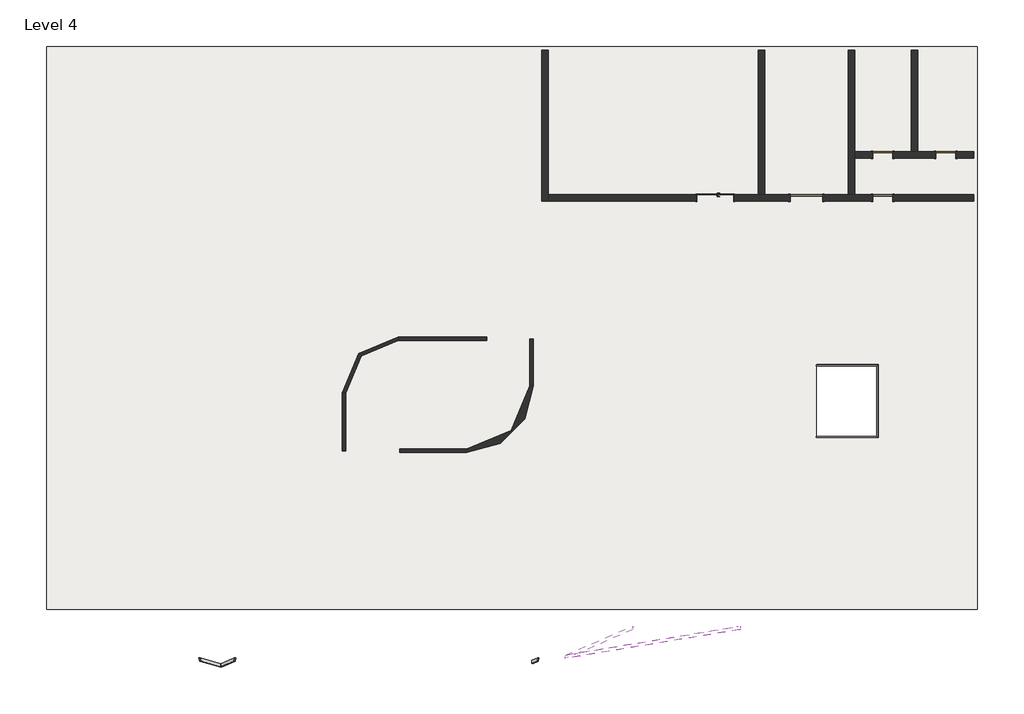
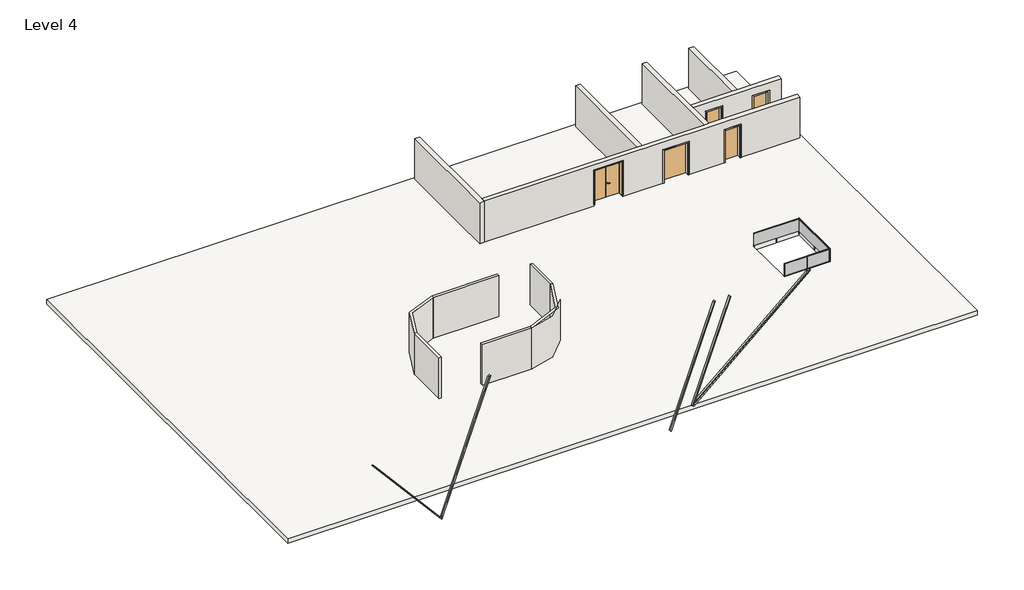
# One storey: 12 walls, 6 members, 5 doors, 1 railing, 1 slab.
"""IFC4 building model written with IfcOpenShell, lengths in millimetres."""

import ifcopenshell
import ifcopenshell.guid

model = None  # the IFC model being written
_history = None  # IfcOwnerHistory: only IFC2X3 demands one
_inside = {}  # id of a spatial element -> (the spatial element, [elements in it])
_under = {}  # id of a project, library or spatial element -> (it, [spatial elements below it])
_declared = {}  # id of a project -> (the project, [libraries it declares])
_typed = {}  # id of a type object -> (the type object, [elements of that type])
_made_of = {}  # id of a material, layer set ... -> (it, [elements and type objects made of it])


def new_model(schema):
    """Start an empty IFC model of exactly this schema.

    Asked for "IFC4X3", IfcOpenShell would pick the latest addendum, in which some entities
    have other attributes; the version numbers below select the first issue.
    IFC2X3 requires an IfcOwnerHistory on every rooted entity: one is made here for all.
    """
    global model, _history
    if schema == "IFC4X3":
        model = ifcopenshell.file(schema_version=(4, 3, 0, 0))
    else:
        model = ifcopenshell.file(schema=schema)
    _inside.clear()
    _under.clear()
    _declared.clear()
    _typed.clear()
    _made_of.clear()
    _history = None
    if model.schema == "IFC2X3":
        org = make("IfcOrganization", Name="unknown")
        user = make(
            "IfcPersonAndOrganization",
            ThePerson=make("IfcPerson", FamilyName="unknown"),
            TheOrganization=org,
        )
        app = make(
            "IfcApplication",
            ApplicationDeveloper=org,
            Version="unknown",
            ApplicationFullName="unknown",
            ApplicationIdentifier="unknown",
        )
        _history = make(
            "IfcOwnerHistory",
            OwningUser=user,
            OwningApplication=app,
            ChangeAction="ADDED",
            CreationDate=0,
        )
    return model


def make(cls, **values):
    """One entity of the class cls with the attributes given. An attribute that is None is left unset."""
    return model.create_entity(
        cls, **{name: value for name, value in values.items() if value is not None}
    )


def rooted(cls, **values):
    """An entity with a GlobalId (a new one), such as an element, a storey or a relation."""
    return make(cls, GlobalId=ifcopenshell.guid.new(), OwnerHistory=_history, **values)


def si_unit(unit_type, name, prefix=None):
    """IfcSIUnit, for example si_unit("LENGTHUNIT", "METRE", prefix="MILLI")."""
    return make("IfcSIUnit", UnitType=unit_type, Prefix=prefix, Name=name)


def assignment(units):
    """IfcUnitAssignment: the units of a project."""
    return None if units is None else make("IfcUnitAssignment", Units=units)


def point(xyz):
    """IfcCartesianPoint."""
    return None if xyz is None else make("IfcCartesianPoint", Coordinates=xyz)


def direction(xyz):
    """IfcDirection."""
    return None if xyz is None else make("IfcDirection", DirectionRatios=xyz)


def frame(location, z_axis=None, x_axis=None):
    """IfcAxis2Placement3D, a coordinate frame: its origin and axes. An axis left out is left unset."""
    return make(
        "IfcAxis2Placement3D",
        Location=point(location),
        Axis=direction(z_axis),
        RefDirection=direction(x_axis),
    )


def frame_2d(location, x_axis=None):
    """IfcAxis2Placement2D, a coordinate frame in the plane: its origin and x axis."""
    return make(
        "IfcAxis2Placement2D", Location=point(location), RefDirection=direction(x_axis)
    )


def origin():
    """The frame at (0, 0, 0) with its axes left unset."""
    return frame((0.0, 0.0, 0.0))


def origin_with_axes():
    """The frame at (0, 0, 0) with the z axis (0, 0, 1) and the x axis (1, 0, 0) written out."""
    return frame((0.0, 0.0, 0.0), z_axis=(0.0, 0.0, 1.0), x_axis=(1.0, 0.0, 0.0))


def place(relative_to, where):
    """IfcLocalPlacement: puts the frame where relative to a parent placement (None: the world)."""
    return make(
        "IfcLocalPlacement", PlacementRelTo=relative_to, RelativePlacement=where
    )


def context(
    kind, dimensions, precision=None, world=None, true_north=None, identifier=None
):
    """IfcGeometricRepresentationContext, for example the 3D "Model" context."""
    return make(
        "IfcGeometricRepresentationContext",
        ContextIdentifier=identifier,
        ContextType=kind,
        CoordinateSpaceDimension=dimensions,
        Precision=precision,
        WorldCoordinateSystem=world,
        TrueNorth=true_north,
    )


def project(units=None, contexts=None):
    """IfcProject with its units and contexts."""
    return rooted(
        "IfcProject",
        Name="project",
        RepresentationContexts=contexts,
        UnitsInContext=assignment(units),
    )


def spatial(cls, under=None, at=None, **own):
    """A site, building, storey or space (cls), placed at a placement, below another one or the project."""
    s = rooted(cls, ObjectPlacement=at, **own)
    if under is not None:
        _under.setdefault(under.id(), (under, []))[1].append(s)
    return s


def polyline(points):
    """IfcPolyline through the points."""
    return make("IfcPolyline", Points=[point(p) for p in points])


def circle_curve(where, radius):
    """IfcCircle in the frame where."""
    return make("IfcCircle", Position=where, Radius=radius)


def ellipse_curve(where, semi_axis1, semi_axis2):
    """IfcEllipse in the frame where."""
    return make(
        "IfcEllipse", Position=where, SemiAxis1=semi_axis1, SemiAxis2=semi_axis2
    )


def trimmed(basis, trim1, trim2, sense, master):
    """IfcTrimmedCurve: the piece of a basis curve between two trims."""
    return make(
        "IfcTrimmedCurve",
        BasisCurve=basis,
        Trim1=trim1,
        Trim2=trim2,
        SenseAgreement=sense,
        MasterRepresentation=master,
    )


def segment(curve, same_sense, transition):
    """IfcCompositeCurveSegment."""
    return make(
        "IfcCompositeCurveSegment",
        Transition=transition,
        SameSense=same_sense,
        ParentCurve=curve,
    )


def composite_curve(segments, self_intersect=None):
    """IfcCompositeCurve: segments joined end to end."""
    return make("IfcCompositeCurve", Segments=segments, SelfIntersect=self_intersect)


def outline(outer, holes=None, kind="AREA"):
    """IfcArbitraryClosedProfileDef: a profile drawn as a closed curve; with holes, ...WithVoids."""
    if holes is None:
        return make("IfcArbitraryClosedProfileDef", ProfileType=kind, OuterCurve=outer)
    return make(
        "IfcArbitraryProfileDefWithVoids",
        ProfileType=kind,
        OuterCurve=outer,
        InnerCurves=holes,
    )


def extrude(swept, where, along, depth):
    """IfcExtrudedAreaSolid: the profile swept, set in the frame where, extruded along a direction by depth."""
    return make(
        "IfcExtrudedAreaSolid",
        SweptArea=swept,
        Position=where,
        ExtrudedDirection=direction(along),
        Depth=depth,
    )


def faces_of(points, faces, orient=None, outer=None):
    """IfcFace entities. A face is a list of loops; a loop is a list of indices into points, from 0.

    orient and outer hold one flag for each loop. By default every Orientation is true, the
    first loop of a face is its IfcFaceOuterBound and the others are IfcFaceBound.
    """
    made = []
    for i, loops in enumerate(faces):
        bounds = []
        for j, loop in enumerate(loops):
            is_outer = j == 0 if outer is None else outer[i][j]
            bounds.append(
                make(
                    "IfcFaceOuterBound" if is_outer else "IfcFaceBound",
                    Bound=make("IfcPolyLoop", Polygon=[points[k] for k in loop]),
                    Orientation=True if orient is None else orient[i][j],
                )
            )
        made.append(make("IfcFace", Bounds=bounds))
    return made


def faceted_brep(points, faces, orient=None, outer=None, voids=None):
    """IfcFacetedBrep: a solid bounded by flat faces; with voids (closed shells), ...WithVoids."""
    shared = [point(p) for p in points]
    hull = make("IfcClosedShell", CfsFaces=faces_of(shared, faces, orient, outer))
    if voids is None:
        return make("IfcFacetedBrep", Outer=hull)
    return make(
        "IfcFacetedBrepWithVoids",
        Outer=hull,
        Voids=[
            make(cls, CfsFaces=faces_of(shared, fs, o, b)) for cls, fs, o, b in voids
        ],
    )


def shape(context_of_items, identifier, shape_type, items):
    """IfcShapeRepresentation: the items that make up one representation, for example the "Body"."""
    return make(
        "IfcShapeRepresentation",
        ContextOfItems=context_of_items,
        RepresentationIdentifier=identifier,
        RepresentationType=shape_type,
        Items=items,
    )


def source(mapping_origin, context_of_items, identifier, shape_type, items):
    """IfcRepresentationMap: a shape defined once, which mapped items show again and again."""
    return make(
        "IfcRepresentationMap",
        MappingOrigin=mapping_origin,
        MappedRepresentation=shape(context_of_items, identifier, shape_type, items),
    )


def transform(
    local_origin,
    x_axis=None,
    y_axis=None,
    z_axis=None,
    scale=None,
    scale2=None,
    scale3=None,
    uniform=True,
):
    """IfcCartesianTransformationOperator3D, or its non-uniform kind. x_axis, y_axis, z_axis: its Axis1, 2, 3."""
    if uniform:
        return make(
            "IfcCartesianTransformationOperator3D",
            Axis1=direction(x_axis),
            Axis2=direction(y_axis),
            LocalOrigin=point(local_origin),
            Scale=scale,
            Axis3=direction(z_axis),
        )
    return make(
        "IfcCartesianTransformationOperator3DnonUniform",
        Axis1=direction(x_axis),
        Axis2=direction(y_axis),
        LocalOrigin=point(local_origin),
        Scale=scale,
        Axis3=direction(z_axis),
        Scale2=scale2,
        Scale3=scale3,
    )


def mapped(mapping_source, mapping_target):
    """IfcMappedItem: shows the shape of a source again, moved by a transform."""
    return make(
        "IfcMappedItem", MappingSource=mapping_source, MappingTarget=mapping_target
    )


def made_of(thing, what):
    """Note that an element or type object is made of a material, layer set ...; save() writes the relation."""
    if what is not None:
        _made_of.setdefault(what.id(), (what, []))[1].append(thing)
    return thing


def element(
    cls,
    number,
    at=None,
    inside=None,
    cuts=None,
    type_object=None,
    material=None,
    context=None,
    identifier="Body",
    shape_type=None,
    held_by="IfcProductDefinitionShape",
    body=None,
    shapes=None,
    **own,
):
    """One element of the class cls, such as IfcWall. Its Tag is "e" and its number.

    at: its placement. inside: the storey or other place that contains it. cuts: it is an
    opening in that element (IfcRelVoidsElement). A single representation is given by context,
    identifier, shape_type and body (its items); several are given by shapes. held_by: the class
    of the entity that holds the representations. save() writes the other relations.
    """
    e = rooted(cls, Tag="e%d" % number, ObjectPlacement=at, **own)
    if body is not None:
        shapes = [shape(context, identifier, shape_type, body)]
    if shapes is not None:
        e.Representation = make(held_by, Representations=shapes)
    if inside is not None:
        _inside.setdefault(inside.id(), (inside, []))[1].append(e)
    if cuts is not None:
        rooted(
            "IfcRelVoidsElement", RelatingBuildingElement=cuts, RelatedOpeningElement=e
        )
    if type_object is not None:
        _typed.setdefault(type_object.id(), (type_object, []))[1].append(e)
    return made_of(e, material)


def aggregate(whole, parts):
    """IfcRelAggregates: a whole, such as a stair, and the parts it consists of."""
    return rooted("IfcRelAggregates", RelatingObject=whole, RelatedObjects=parts)


def save(model, path):
    """Write the relations noted so far, then the file.

    IfcRelAggregates (storeys below a building ...), IfcRelContainedInSpatialStructure (elements
    in a storey), IfcRelDefinesByType, IfcRelAssociatesMaterial and IfcRelDeclares: one each for
    every whole, place, type object, material and project.
    """
    for whole, parts in _under.values():
        aggregate(whole, parts)
    for where, things in _inside.values():
        rooted(
            "IfcRelContainedInSpatialStructure",
            RelatedElements=things,
            RelatingStructure=where,
        )
    for kind, things in _typed.values():
        rooted("IfcRelDefinesByType", RelatedObjects=things, RelatingType=kind)
    for what, things in _made_of.values():
        rooted("IfcRelAssociatesMaterial", RelatedObjects=things, RelatingMaterial=what)
    for by, libraries in _declared.values():
        rooted("IfcRelDeclares", RelatingContext=by, RelatedDefinitions=libraries)
    model.write(path)


def plane_surface(at):
    """IfcPlane: the flat surface through the origin of the frame at, square to its z axis."""
    return make("IfcPlane", Position=at)


def cylinder_surface(at, radius):
    """IfcCylindricalSurface: all points at the distance radius from the z axis of the frame at."""
    return make("IfcCylindricalSurface", Position=at, Radius=radius)


def advanced_brep(points, edges, surfaces, faces):
    """IfcAdvancedBrep: a solid bounded by faces that lie on surfaces and meet in shared edges.

    An edge is (start, end): straight between two places in points (the first is 0);
    or (start, end, curve); or (start, end, curve, False) where it runs against its curve.
    A face is (place in surfaces, loops), or (place, loops, False) where it looks against
    its surface's normal. A loop lists edges by number (the first is 1), with a minus sign
    where the edge is run from its end to its start. The first loop is the outer one.
    """
    corners = [point(p) for p in points]
    vertices = [make("IfcVertexPoint", VertexGeometry=c) for c in corners]
    made = []
    for start, end, *more in edges:
        made.append(
            make(
                "IfcEdgeCurve",
                EdgeStart=vertices[start],
                EdgeEnd=vertices[end],
                EdgeGeometry=more[0] if more else make("IfcPolyline", Points=[corners[start], corners[end]]),
                SameSense=more[1] if len(more) > 1 else True,
            )
        )
    hull = []
    for where, loops, *sense in faces:
        bounds = []
        for j, loop in enumerate(loops):
            ring = [make("IfcOrientedEdge", EdgeElement=made[abs(k) - 1], Orientation=k > 0) for k in loop]
            bounds.append(
                make(
                    "IfcFaceOuterBound" if j == 0 else "IfcFaceBound",
                    Bound=make("IfcEdgeLoop", EdgeList=ring),
                    Orientation=True,
                )
            )
        hull.append(make("IfcAdvancedFace", Bounds=bounds, FaceSurface=surfaces[where], SameSense=sense[0] if sense else True))
    return make("IfcAdvancedBrep", Outer=make("IfcClosedShell", CfsFaces=hull))


def door_double_flush_variable_door_double_flush_variable_ac6c3b87(model_context):
    return source(origin(), model_context, "Body", "SolidModel", [
        advanced_brep(
        [(90.0, 139.4346141, 1000.0), (110.0, 139.4346141, 1000.0), (90.0, 69.4346141, 1000.0), (110.0, 89.4346141, 1000.0), (220.0, 69.4346141, 1000.0), (220.0, 89.4346141, 1000.0)],
        [
            (0, 1, circle_curve(frame((100.0, 139.4346141, 1000.0), z_axis=(0.0, 1.0, 0.0), x_axis=(1.0, 0.0, 0.0)), 10.0)),
            (1, 0, circle_curve(frame((100.0, 139.4346141, 1000.0), z_axis=(0.0, 1.0, 0.0), x_axis=(1.0, 0.0, 0.0)), 10.0)),
            (0, 2),
            (2, 3, ellipse_curve(frame((100.0, 79.4346141, 1000.0), z_axis=(-0.7071067811865385, 0.7071067811865565, 0.0), x_axis=(0.7071067811865563, 0.7071067811865386, 0.0)), 14.1421356, 10.0)),
            (3, 1),
            (3, 2, ellipse_curve(frame((100.0, 79.4346141, 1000.0), z_axis=(-0.7071067811865385, 0.7071067811865565, 0.0), x_axis=(0.7071067811865563, 0.7071067811865386, 0.0)), 14.1421356, 10.0)),
            (4, 5, circle_curve(frame((220.0, 79.4346141, 1000.0), z_axis=(1.0, 0.0, 0.0), x_axis=(0.0, 1.0, 0.0)), 10.0)),
            (5, 4, circle_curve(frame((220.0, 79.4346141, 1000.0), z_axis=(1.0, 0.0, 0.0), x_axis=(0.0, 1.0, 0.0)), 10.0)),
            (2, 4),
            (5, 3),
        ],
        [
            plane_surface(frame((100.0, 139.4346141, -287.7526403), z_axis=(0.0, 1.0, 0.0), x_axis=(0.0, 0.0, 1.0))),
            cylinder_surface(frame((100.0, 139.4346141, 1000.0), z_axis=(0.0, 1.0, 0.0), x_axis=(1.0, 0.0, 0.0)), 10.0),
            plane_surface(frame((220.0, 79.4346141, -287.7526403), z_axis=(1.0, 0.0, 0.0), x_axis=(0.0, 0.0, 1.0))),
            cylinder_surface(frame((100.0, 79.4346141, 1000.0), z_axis=(-1.0, 0.0, 0.0), x_axis=(0.0, 1.0, 0.0)), 10.0),
        ],
        [
            (0, [[1, 2]]),
            (1, [[-1, 3, 4, 5]]),
            (1, [[-2, -5, 6, -3]]),
            (2, [[7, 8]]),
            (3, [[-4, 9, -8, 10]]),
            (3, [[-6, -10, -7, -9]]),
        ],
    ),
        advanced_brep(
        [(110.0, 199.4346141, 1000.0), (90.0, 199.4346141, 1000.0), (110.0, 229.4346141, 1000.0), (90.0, 249.4346141, 1000.0), (220.0, 229.4346141, 1000.0), (220.0, 249.4346141, 1000.0)],
        [
            (0, 1, circle_curve(frame((100.0, 199.4346141, 1000.0), z_axis=(0.0, -1.0, 0.0), x_axis=(-1.0, 0.0, 0.0)), 10.0)),
            (1, 0, circle_curve(frame((100.0, 199.4346141, 1000.0), z_axis=(0.0, -1.0, 0.0), x_axis=(-1.0, 0.0, 0.0)), 10.0)),
            (0, 2),
            (2, 3, ellipse_curve(frame((100.0, 239.4346141, 1000.0), z_axis=(-0.7071067811865475, -0.7071067811865475, 0.0), x_axis=(0.7071067811865474, -0.7071067811865476, 0.0)), 14.1421356, 10.0)),
            (3, 1),
            (3, 2, ellipse_curve(frame((100.0, 239.4346141, 1000.0), z_axis=(-0.7071067811865475, -0.7071067811865475, 0.0), x_axis=(0.7071067811865474, -0.7071067811865476, 0.0)), 14.1421356, 10.0)),
            (4, 5, circle_curve(frame((220.0, 239.4346141, 1000.0), z_axis=(1.0, 0.0, 0.0), x_axis=(0.0, 1.0, 0.0)), 10.0)),
            (5, 4, circle_curve(frame((220.0, 239.4346141, 1000.0), z_axis=(1.0, 0.0, 0.0), x_axis=(0.0, 1.0, 0.0)), 10.0)),
            (2, 4),
            (5, 3),
        ],
        [
            plane_surface(frame((100.0, 199.4346141, -287.7526403), z_axis=(0.0, -1.0, 0.0), x_axis=(0.0, 0.0, 1.0))),
            cylinder_surface(frame((100.0, 199.4346141, 1000.0), z_axis=(0.0, -1.0, 0.0), x_axis=(-1.0, 0.0, 0.0)), 10.0),
            plane_surface(frame((220.0, 239.4346141, -287.7526403), z_axis=(1.0, 0.0, 0.0), x_axis=(0.0, 0.0, 1.0))),
            cylinder_surface(frame((100.0, 239.4346141, 1000.0), z_axis=(-1.0, 0.0, 0.0), x_axis=(0.0, 1.0, 0.0)), 10.0),
        ],
        [
            (0, [[1, 2]]),
            (1, [[-1, 3, 4, 5]]),
            (1, [[-2, -5, 6, -3]]),
            (2, [[7, 8]]),
            (3, [[-4, 9, -8, 10]]),
            (3, [[-6, -10, -7, -9]]),
        ],
    ),
        extrude(outline(composite_curve([segment(trimmed(circle_curve(frame_2d((1000.0, 100.0)), 20.0), [point((1000.0, 80.0))], [point((1000.0, 120.0))], False, "CARTESIAN"), True, "CONTINUOUS"), segment(trimmed(circle_curve(frame_2d((1000.0, 100.0)), 20.0), [point((1000.0, 120.0))], [point((1000.0, 80.0))], False, "CARTESIAN"), True, "CONTINUOUS")], self_intersect=False)), frame((0.0, 129.4346141, 0.0), z_axis=(0.0, 1.0, 0.0), x_axis=(0.0, 0.0, 1.0)), (0.0, 0.0, 1.0), 10.0),
        extrude(outline(composite_curve([segment(trimmed(circle_curve(frame_2d((1000.0, 100.0)), 20.0), [point((1000.0, 80.0))], [point((1000.0, 120.0))], False, "CARTESIAN"), True, "CONTINUOUS"), segment(trimmed(circle_curve(frame_2d((1000.0, 100.0)), 20.0), [point((1000.0, 120.0))], [point((1000.0, 80.0))], False, "CARTESIAN"), True, "CONTINUOUS")], self_intersect=False)), frame((0.0, 189.4346141, 0.0), z_axis=(0.0, 1.0, 0.0), x_axis=(0.0, 0.0, 1.0)), (0.0, 0.0, 1.0), 10.0),
        extrude(outline(polyline([(0.0, 164.4346141), (-871.25, 164.4346141), (-871.25, 189.4346141), (0.0, 189.4346141), (0.0, 164.4346141)])), frame((0.0, 0.0, 100.0), z_axis=(0.0, 0.0, 1.0), x_axis=(1.0, 0.0, 0.0)), (0.0, 0.0, 1.0), 2250.0),
        extrude(outline(polyline([(871.25, 164.4346141), (0.0, 164.4346141), (0.0, 189.4346141), (871.25, 189.4346141), (871.25, 164.4346141)])), frame((0.0, 0.0, 100.0), z_axis=(0.0, 0.0, 1.0), x_axis=(1.0, 0.0, 0.0)), (0.0, 0.0, 1.0), 2250.0),
        faceted_brep([(905.75, -150.5653859, 100.0), (856.25, -150.5653859, 100.0), (856.25, 164.4346141, 100.0), (871.25, 164.4346141, 100.0), (871.25, 189.4346141, 100.0), (905.75, 189.4346141, 100.0), (905.75, 164.4346141, 100.0), (900.75, 164.4346141, 100.0), (900.75, 184.4346141, 100.0), (876.25, 184.4346141, 100.0), (876.25, 159.4346141, 100.0), (861.25, 159.4346141, 100.0), (861.25, -145.5653859, 100.0), (900.75, -145.5653859, 100.0), (900.75, -135.5653859, 100.0), (905.75, -135.5653859, 100.0), (905.75, -150.5653859, 2384.5), (-905.75, -150.5653859, 2384.5), (-905.75, -150.5653859, 100.0), (-856.25, -150.5653859, 100.0), (-856.25, -150.5653859, 2335.0), (856.25, -150.5653859, 2335.0), (856.25, 164.4346141, 2335.0), (-856.25, 164.4346141, 2335.0), (-856.25, 164.4346141, 100.0), (-871.25, 164.4346141, 100.0), (-871.25, 164.4346141, 2350.0), (871.25, 164.4346141, 2350.0), (871.25, 189.4346141, 2350.0), (-871.25, 189.4346141, 2350.0), (-871.25, 189.4346141, 100.0), (-905.75, 189.4346141, 100.0), (-905.75, 189.4346141, 2384.5), (905.75, 189.4346141, 2384.5), (905.75, 164.4346141, 2384.5), (-905.75, 164.4346141, 2384.5), (-905.75, 164.4346141, 100.0), (-900.75, 164.4346141, 100.0), (-900.75, 164.4346141, 2379.5), (900.75, 164.4346141, 2379.5), (900.75, 184.4346141, 2379.5), (-900.75, 184.4346141, 2379.5), (-900.75, 184.4346141, 100.0), (-876.25, 184.4346141, 100.0), (-876.25, 184.4346141, 2355.0), (876.25, 184.4346141, 2355.0), (876.25, 159.4346141, 2355.0), (-876.25, 159.4346141, 2355.0), (-876.25, 159.4346141, 100.0), (-861.25, 159.4346141, 100.0), (-861.25, 159.4346141, 2340.0), (861.25, 159.4346141, 2340.0), (861.25, -145.5653859, 2340.0), (-861.25, -145.5653859, 2340.0), (-861.25, -145.5653859, 100.0), (-900.75, -145.5653859, 100.0), (-900.75, -145.5653859, 2379.5), (900.75, -145.5653859, 2379.5), (900.75, -135.5653859, 2379.5), (-900.75, -135.5653859, 2379.5), (-900.75, -135.5653859, 100.0), (-905.75, -135.5653859, 100.0), (-905.75, -135.5653859, 2384.5), (905.75, -135.5653859, 2384.5)], [[[0, 1, 2, 3, 4, 5, 6, 7, 8, 9, 10, 11, 12, 13, 14, 15]], [[1, 0, 16, 17, 18, 19, 20, 21]], [[2, 1, 21, 22]], [[3, 2, 22, 23, 24, 25, 26, 27]], [[4, 3, 27, 28]], [[5, 4, 28, 29, 30, 31, 32, 33]], [[6, 5, 33, 34]], [[7, 6, 34, 35, 36, 37, 38, 39]], [[8, 7, 39, 40]], [[9, 8, 40, 41, 42, 43, 44, 45]], [[10, 9, 45, 46]], [[11, 10, 46, 47, 48, 49, 50, 51]], [[12, 11, 51, 52]], [[13, 12, 52, 53, 54, 55, 56, 57]], [[14, 13, 57, 58]], [[15, 14, 58, 59, 60, 61, 62, 63]], [[0, 15, 63, 16]], [[17, 62, 61, 18]], [[18, 61, 60, 55, 54, 49, 48, 43, 42, 37, 36, 31, 30, 25, 24, 19]], [[23, 20, 19, 24]], [[29, 26, 25, 30]], [[35, 32, 31, 36]], [[41, 38, 37, 42]], [[47, 44, 43, 48]], [[53, 50, 49, 54]], [[59, 56, 55, 60]], [[22, 21, 20, 23]], [[28, 27, 26, 29]], [[34, 33, 32, 35]], [[40, 39, 38, 41]], [[46, 45, 44, 47]], [[52, 51, 50, 53]], [[58, 57, 56, 59]], [[16, 63, 62, 17]]]),
    ])


def m_single_flush_0915_x_2134mm_1c84716f(model_context):
    return source(origin(), model_context, "Body", "SweptSolid", [
        extrude(outline(polyline([(2210.0, -533.5), (0.0, -533.5), (0.0, -457.5), (2134.0, -457.5), (2134.0, 457.5), (0.0, 457.5), (0.0, 533.5), (2210.0, 533.5), (2210.0, -533.5)])), frame((0.0, -175.0, 0.0), z_axis=(0.0, 1.0, 0.0), x_axis=(0.0, 0.0, 1.0)), (0.0, 0.0, 1.0), 25.0),
        extrude(outline(polyline([(2210.0, 533.5), (2210.0, -533.5), (0.0, -533.5), (0.0, -457.5), (2134.0, -457.5), (2134.0, 457.5), (0.0, 457.5), (0.0, 533.5), (2210.0, 533.5)])), frame((0.0, 150.0, 0.0), z_axis=(0.0, 1.0, 0.0), x_axis=(0.0, 0.0, 1.0)), (0.0, 0.0, 1.0), 25.0),
        extrude(outline(polyline([(457.5, -99.0), (457.5, -150.0), (-457.5, -150.0), (-457.5, -99.0), (457.5, -99.0)])), origin_with_axes(), (0.0, 0.0, 1.0), 2134.0),
    ])


def m_single_flush_1500_x_2134mm_2_edebd810(model_context):
    return source(origin(), model_context, "Body", "SweptSolid", [
        extrude(outline(polyline([(2210.0, -826.0), (0.0, -826.0), (0.0, -750.0), (2134.0, -750.0), (2134.0, 750.0), (0.0, 750.0), (0.0, 826.0), (2210.0, 826.0), (2210.0, -826.0)])), frame((0.0, -175.0, 0.0), z_axis=(0.0, 1.0, 0.0), x_axis=(0.0, 0.0, 1.0)), (0.0, 0.0, 1.0), 25.0),
        extrude(outline(polyline([(2210.0, 826.0), (2210.0, -826.0), (0.0, -826.0), (0.0, -750.0), (2134.0, -750.0), (2134.0, 750.0), (0.0, 750.0), (0.0, 826.0), (2210.0, 826.0)])), frame((0.0, 150.0, 0.0), z_axis=(0.0, 1.0, 0.0), x_axis=(0.0, 0.0, 1.0)), (0.0, 0.0, 1.0), 25.0),
        extrude(outline(polyline([(750.0, -99.0), (750.0, -150.0), (-750.0, -150.0), (-750.0, -99.0), (750.0, -99.0)])), origin_with_axes(), (0.0, 0.0, 1.0), 2134.0),
    ])


def rectangular_mullion_50_x_150mm_6888afb9(model_context):
    return source(origin(), model_context, "Body", "SweptSolid", [
        extrude(outline(polyline([(0.0, 0.0), (-85.321119, -50.0), (-8217.0308307, -50.0), (-8288.6527046, 0.0), (0.0, 0.0)])), frame((0.0, -75.0, 0.0), z_axis=(0.0, 1.0, 0.0), x_axis=(0.0, 0.0, 1.0)), (0.0, 0.0, 1.0), 150.0),
    ])


def rectangular_mullion_50_x_150mm_7805e086(model_context):
    return source(origin(), model_context, "Body", "SweptSolid", [
        extrude(outline(polyline([(0.0, 0.0), (-85.321119, -50.0), (-7488.5336568, -50.0), (-7500.253691, 0.0), (0.0, 0.0)])), frame((0.0, -75.0, 0.0), z_axis=(0.0, 1.0, 0.0), x_axis=(0.0, 0.0, 1.0)), (0.0, 0.0, 1.0), 150.0),
    ])


def rectangular_mullion_50_x_150mm_3e1f935b(model_context):
    return source(origin(), model_context, "Body", "SweptSolid", [
        extrude(outline(polyline([(0.0, 0.0), (-213.3099575, -50.0), (-6299.3378645, -50.0), (-6328.6389336, 0.0), (0.0, 0.0)])), frame((0.0, -75.0, 0.0), z_axis=(0.0, 1.0, 0.0), x_axis=(0.0, 0.0, 1.0)), (0.0, 0.0, 1.0), 150.0),
    ])


def rectangular_mullion_50_x_150mm_2c60866a(model_context):
    return source(origin(), model_context, "Body", "SweptSolid", [
        extrude(outline(polyline([(0.0, 0.0), (-71.6218739, -50.0), (-5613.3621531, -50.0), (-5648.2676905, 0.0), (0.0, 0.0)])), frame((0.0, -75.0, 0.0), z_axis=(0.0, 1.0, 0.0), x_axis=(0.0, 0.0, 1.0)), (0.0, 0.0, 1.0), 150.0),
    ])


def rectangular_mullion_50_x_150mm_3d64617b(model_context):
    return source(origin(), model_context, "Body", "SweptSolid", [
        extrude(outline(polyline([(0.0, 0.0), (-11.7094446, -50.0), (-9724.6362561, -50.0), (-9783.1614006, 0.0), (0.0, 0.0)])), frame((0.0, -75.0, 0.0), z_axis=(0.0, 1.0, 0.0), x_axis=(0.0, 0.0, 1.0)), (0.0, 0.0, 1.0), 150.0),
    ])


def rectangular_mullion_50_x_150mm_375b3459(model_context):
    return source(origin(), model_context, "Body", "SweptSolid", [
        extrude(outline(polyline([(0.0, 0.0), (-161.7316361, -50.0), (-9569.8514431, -50.0), (-9783.1614006, 0.0), (0.0, 0.0)])), frame((0.0, -75.0, 0.0), z_axis=(0.0, 1.0, 0.0), x_axis=(0.0, 0.0, 1.0)), (0.0, 0.0, 1.0), 150.0),
    ])


def glas_mpk_39525c5c(model_context):
    return source(origin(), model_context, "Body", "SolidModel", [
        faceted_brep([(28810.8437289, 1285.374085, 9843.2628643), (28810.8437289, 1235.374085, 9843.2628643), (28810.8437289, 1235.374085, 9856.7371357), (28810.8437289, 1285.374085, 9856.7371357), (31650.8437289, 1285.374085, 9843.2628643), (31600.8437289, 1235.374085, 9843.2628643), (31600.8437289, 1235.374085, 9856.7371357), (31650.8437289, 1285.374085, 9856.7371357), (31650.8437289, -2055.3552612, 9843.2628643), (31600.8437289, -2005.3552612, 9843.2628643), (31600.8437289, -2005.3552612, 9856.7371357), (31650.8437289, -2055.3552612, 9856.7371357), (28810.8437289, -2055.3552612, 9843.2628643), (28810.8437289, -2055.3552612, 9856.7371357), (28810.8437289, -2005.3552612, 9856.7371357), (28810.8437289, -2005.3552612, 9843.2628643)], [[[0, 1, 2, 3]], [[1, 0, 4, 5]], [[2, 1, 5, 6]], [[3, 2, 6, 7]], [[0, 3, 7, 4]], [[5, 4, 8, 9]], [[6, 5, 9, 10]], [[7, 6, 10, 11]], [[4, 7, 11, 8]], [[12, 13, 14, 15]], [[9, 8, 12, 15]], [[10, 9, 15, 14]], [[11, 10, 14, 13]], [[8, 11, 13, 12]]]),
        faceted_brep([(28810.8437289, 1245.374085, 9842.8769824), (28810.8437289, 1259.566209, 9842.8769824), (28810.8437289, 1259.566209, 9042.8769824), (28810.8437289, 1245.374085, 9042.8769824), (31610.8437289, 1245.374085, 9842.8769824), (31625.0358529, 1259.566209, 9842.8769824), (31625.0358529, 1259.566209, 9042.8769824), (31610.8437289, 1245.374085, 9042.8769824), (31610.8437289, -2015.3552612, 9842.8769824), (31625.0358529, -2029.5473852, 9842.8769824), (31625.0358529, -2029.5473852, 9042.8769824), (31610.8437289, -2015.3552612, 9042.8769824), (28810.8437289, -2015.3552612, 9842.8769824), (28810.8437289, -2015.3552612, 9042.8769824), (28810.8437289, -2029.5473852, 9042.8769824), (28810.8437289, -2029.5473852, 9842.8769824)], [[[0, 1, 2, 3]], [[1, 0, 4, 5]], [[2, 1, 5, 6]], [[3, 2, 6, 7]], [[0, 3, 7, 4]], [[5, 4, 8, 9]], [[6, 5, 9, 10]], [[7, 6, 10, 11]], [[4, 7, 11, 8]], [[12, 13, 14, 15]], [[9, 8, 12, 15]], [[10, 9, 15, 14]], [[11, 10, 14, 13]], [[8, 11, 13, 12]]]),
        extrude(outline(polyline([(30242.0937289, -2030.3552612), (30242.0937289, -2055.3552612), (30217.0937289, -2055.3552612), (30217.0937289, -2030.3552612), (30242.0937289, -2030.3552612)])), frame((0.0, 0.0, 8800.0), z_axis=(0.0, 0.0, 1.0), x_axis=(1.0, 0.0, 0.0)), (0.0, 0.0, 1.0), 1043.2628643),
        extrude(outline(polyline([(31625.8437289, -372.4905881), (31650.8437289, -372.4905881), (31650.8437289, -397.4905881), (31625.8437289, -397.4905881), (31625.8437289, -372.4905881)])), frame((0.0, 0.0, 8800.0), z_axis=(0.0, 0.0, 1.0), x_axis=(1.0, 0.0, 0.0)), (0.0, 0.0, 1.0), 1043.2628643),
        extrude(outline(polyline([(30217.0937289, 1260.374085), (30217.0937289, 1285.374085), (30242.0937289, 1285.374085), (30242.0937289, 1260.374085), (30217.0937289, 1260.374085)])), frame((0.0, 0.0, 8800.0), z_axis=(0.0, 0.0, 1.0), x_axis=(1.0, 0.0, 0.0)), (0.0, 0.0, 1.0), 1043.2628643),
        extrude(outline(polyline([(31625.8437289, -2040.3552612), (31650.8437289, -2040.3552612), (31650.8437289, -2065.3552612), (31625.8437289, -2065.3552612), (31625.8437289, -2040.3552612)])), frame((0.0, 0.0, 8800.0), z_axis=(0.0, 0.0, 1.0), x_axis=(1.0, 0.0, 0.0)), (0.0, 0.0, 1.0), 1043.2628643),
        extrude(outline(polyline([(31635.8437289, 1260.374085), (31635.8437289, 1285.374085), (31660.8437289, 1285.374085), (31660.8437289, 1260.374085), (31635.8437289, 1260.374085)])), frame((0.0, 0.0, 8800.0), z_axis=(0.0, 0.0, 1.0), x_axis=(1.0, 0.0, 0.0)), (0.0, 0.0, 1.0), 1043.2628643),
        extrude(outline(polyline([(28823.3437289, -2030.3552612), (28823.3437289, -2055.3552612), (28798.3437289, -2055.3552612), (28798.3437289, -2030.3552612), (28823.3437289, -2030.3552612)])), frame((0.0, 0.0, 8800.0), z_axis=(0.0, 0.0, 1.0), x_axis=(1.0, 0.0, 0.0)), (0.0, 0.0, 1.0), 1043.2628643),
        extrude(outline(polyline([(28810.8437289, 1260.374085), (28810.8437289, 1285.374085), (28835.8437289, 1285.374085), (28835.8437289, 1260.374085), (28810.8437289, 1260.374085)])), frame((0.0, 0.0, 8800.0), z_axis=(0.0, 0.0, 1.0), x_axis=(1.0, 0.0, 0.0)), (0.0, 0.0, 1.0), 1043.2628643),
    ])


model = new_model("IFC4")

# Units and contexts
model_context = context("Model", 3, world=origin())
ifc_project = project(units=[si_unit("LENGTHUNIT", "METRE", prefix="MILLI")], contexts=[model_context])

# Site, building, storey
site = spatial("IfcSite", under=ifc_project)
building = spatial("IfcBuilding", under=site)
storey = spatial("IfcBuildingStorey", under=building, Name="Level 4", Elevation=9000.0)

# Doors
placement = place(None, origin())
door_double_flush_variable_door_double_flush_variable_shape = door_double_flush_variable_door_double_flush_variable_ac6c3b87(model_context)
element("IfcDoor", 1, ObjectType="Door Double Flush - Variable : Door Double Flush - Variable", at=placement, inside=storey, context=model_context, shape_type="MappedRepresentation", body=[
    mapped(door_double_flush_variable_door_double_flush_variable_shape, transform((24136.7471367, 8984.3231089, 9000.0), x_axis=(1.0, 0.0, 0.0), y_axis=(0.0, 1.0, 0.0), z_axis=(0.0, 0.0, 1.0))),
])
m_single_flush_0915_x_2134mm_shape = m_single_flush_0915_x_2134mm_1c84716f(model_context)
element("IfcDoor", 2, ObjectType="M_Single-Flush : 0915 x 2134mm", at=placement, inside=storey, context=model_context, shape_type="MappedRepresentation", body=[
    mapped(m_single_flush_0915_x_2134mm_shape, transform((34787.1221367, 10998.757723, 9000.0), x_axis=(-1.0, 0.0, 0.0), y_axis=(0.0, -1.0, 0.0), z_axis=(0.0, 0.0, 1.0))),
])
element("IfcDoor", 3, ObjectType="M_Single-Flush : 0915 x 2134mm", at=placement, inside=storey, context=model_context, shape_type="MappedRepresentation", body=[
    mapped(m_single_flush_0915_x_2134mm_shape, transform((31874.3721367, 10998.757723, 9000.0), x_axis=(-1.0, 0.0, 0.0), y_axis=(0.0, -1.0, 0.0), z_axis=(0.0, 0.0, 1.0))),
])
element("IfcDoor", 4, ObjectType="M_Single-Flush : 0915 x 2134mm", at=placement, inside=storey, context=model_context, shape_type="MappedRepresentation", body=[
    mapped(m_single_flush_0915_x_2134mm_shape, transform((31874.3721367, 8998.757723, 9000.0), x_axis=(-1.0, 0.0, 0.0), y_axis=(0.0, -1.0, 0.0), z_axis=(0.0, 0.0, 1.0))),
])
m_single_flush_1500_x_2134mm_2_shape = m_single_flush_1500_x_2134mm_2_edebd810(model_context)
element("IfcDoor", 5, ObjectType="M_Single-Flush : 1500 x 2134mm 2", at=placement, inside=storey, context=model_context, shape_type="MappedRepresentation", body=[
    mapped(m_single_flush_1500_x_2134mm_2_shape, transform((28342.9971367, 8998.757723, 9000.0), x_axis=(-1.0, 0.0, 0.0), y_axis=(0.0, -1.0, 0.0), z_axis=(0.0, 0.0, 1.0))),
])

# Members
rectangular_mullion_50_x_150mm_shape = rectangular_mullion_50_x_150mm_6888afb9(model_context)
element("IfcMember", 6, ObjectType="Rectangular Mullion : 50 x 150mm", at=placement, inside=storey, context=model_context, shape_type="MappedRepresentation", body=[
    mapped(rectangular_mullion_50_x_150mm_shape, transform((5377.8841529, -10856.2576342, 16077.9460567), x_axis=(0.8724314351462178, -0.11823606660145622, -0.4742189615813849), y_axis=(0.0, 0.9702957262759964, -0.24192189559966842), z_axis=(0.48873652510193155, 0.21106026657131102, 0.8465164929912093))),
])
rectangular_mullion_50_x_150mm_2_shape = rectangular_mullion_50_x_150mm_7805e086(model_context)
element("IfcMember", 7, ObjectType="Rectangular Mullion : 50 x 150mm", at=placement, inside=storey, context=model_context, shape_type="MappedRepresentation", body=[
    mapped(rectangular_mullion_50_x_150mm_2_shape, transform((19377.8841529, -10856.2576342, 16077.9460567), x_axis=(0.8724314351462182, -0.118236066601456, -0.474218961581384), y_axis=(0.0, 0.9702957262759963, -0.24192189559966853), z_axis=(0.48873652510193055, 0.21106026657131124, 0.8465164929912097))),
])
rectangular_mullion_50_x_150mm_3_shape = rectangular_mullion_50_x_150mm_3e1f935b(model_context)
element("IfcMember", 8, ObjectType="Rectangular Mullion : 50 x 150mm", at=placement, inside=storey, context=model_context, shape_type="MappedRepresentation", body=[
    mapped(rectangular_mullion_50_x_150mm_3_shape, transform((17207.380392, -12191.9818546, 10720.6488212), x_axis=(-0.8724314351462175, 0.11823606660145633, 0.4742189615813853), y_axis=(0.0, 0.9702957262759964, -0.2419218955996684), z_axis=(-0.488736525101932, -0.21106026657131094, -0.8465164929912091))),
])
rectangular_mullion_50_x_150mm_4_shape = rectangular_mullion_50_x_150mm_2c60866a(model_context)
element("IfcMember", 9, ObjectType="Rectangular Mullion : 50 x 150mm", at=placement, inside=storey, context=model_context, shape_type="MappedRepresentation", body=[
    mapped(rectangular_mullion_50_x_150mm_4_shape, transform((1326.9168323, -12605.6628836, 9061.4648376), x_axis=(-0.7594865733990562, -0.15737575195413048, -0.6311996653384983), y_axis=(0.0, 0.9702957262759964, -0.2419218955996685), z_axis=(0.6505229779389503, -0.1837364315191979, -0.7369265763331045))),
])
rectangular_mullion_50_x_150mm_5_shape = rectangular_mullion_50_x_150mm_3d64617b(model_context)
element("IfcMember", 10, ObjectType="Rectangular Mullion : 50 x 150mm", at=placement, inside=storey, context=model_context, shape_type="MappedRepresentation", body=[
    mapped(rectangular_mullion_50_x_150mm_5_shape, transform((17207.380392, -12191.9818546, 10720.6488212), x_axis=(-0.5643515799011003, 0.19229756024024097, 0.8028255991115275), y_axis=(-0.004309282844983983, 0.9717923608297846, -0.23579872246099226), z_axis=(-0.8255233033321919, -0.1365329841412873, -0.5476038895926334))),
])
rectangular_mullion_50_x_150mm_6_shape = rectangular_mullion_50_x_150mm_375b3459(model_context)
element("IfcMember", 11, ObjectType="Rectangular Mullion : 50 x 150mm", at=placement, inside=storey, context=model_context, shape_type="MappedRepresentation", body=[
    mapped(rectangular_mullion_50_x_150mm_6_shape, transform((25283.6081085, -10856.2576342, 16077.9460567), x_axis=(0.5643680320991843, -0.19971216240382525, -0.8010017331644683), y_axis=(0.0, 0.9702957262759964, -0.24192189559966856), z_axis=(0.825523303332192, 0.13653298414128745, 0.5476038895926333))),
])

# Railing
glas_mpk_shape = glas_mpk_39525c5c(model_context)
element("IfcRailing", 12, ObjectType="Glas - MPK", at=placement, inside=storey, context=model_context, shape_type="MappedRepresentation", body=[
    mapped(glas_mpk_shape, transform((0.0, 0.0, 0.0), x_axis=(1.0, 0.0, 0.0), y_axis=(0.0, 1.0, 0.0), z_axis=(0.0, 0.0, 1.0))),
])

# Slab
element("IfcSlab", 13, ObjectType="Generic 300mm", at=placement, inside=storey, context=model_context, shape_type="SweptSolid", body=[
    extrude(outline(polyline([(-6732.0028633, 15998.757723), (36243.4971367, 15998.757723), (36243.4971367, -10001.242277), (-6732.0028633, -10001.242277), (-6732.0028633, 15998.757723)]), holes=[polyline([(31663.0737371, 1305.1195288), (28813.0737371, 1305.1195288), (28813.0737371, -2055.6098174), (31663.0737371, -2055.6098174), (31663.0737371, 1305.1195288)])]), frame((0.0, 0.0, 8700.0), z_axis=(0.0, 0.0, 1.0), x_axis=(1.0, 0.0, 0.0)), (0.0, 0.0, 1.0), 300.0),
])

# Walls
element("IfcWall", 14, ObjectType="Generic - 300mm", at=placement, inside=storey, context=model_context, shape_type="Brep", body=[
    faceted_brep([(16117.9971367, 15823.757723, 9000.0), (16117.9971367, 8848.757723, 9000.0), (16117.9971367, 8848.757723, 11700.0), (16117.9971367, 15823.757723, 11700.0), (16417.9971367, 15823.757723, 9000.0), (16417.9971367, 15823.757723, 11700.0), (16417.9971367, 9148.757723, 11700.0), (16417.9971367, 8848.757723, 11700.0), (16417.9971367, 8848.757723, 9000.0), (16417.9971367, 9148.757723, 9000.0)], [[[0, 1, 2, 3]], [[4, 5, 6, 7, 8, 9]], [[1, 0, 4, 9, 8]], [[3, 2, 7, 6, 5]], [[2, 1, 8, 7]], [[0, 3, 5, 4]]]),
])
element("IfcWall", 15, ObjectType="Generic - 300mm", at=placement, inside=storey, context=model_context, shape_type="SweptSolid", body=[
    extrude(outline(polyline([(26117.9971367, 9148.757723), (26117.9971367, 15823.757723), (26417.9971367, 15823.757723), (26417.9971367, 9148.757723), (26117.9971367, 9148.757723)])), frame((0.0, 0.0, 9000.0), z_axis=(0.0, 0.0, 1.0), x_axis=(1.0, 0.0, 0.0)), (0.0, 0.0, 1.0), 2700.0),
])
element("IfcWall", 16, ObjectType="Generic - 300mm", at=placement, inside=storey, context=model_context, shape_type="Brep", body=[
    faceted_brep([(30267.9971367, 15823.757723, 9000.0), (30267.9971367, 9148.757723, 9000.0), (30267.9971367, 9148.757723, 11700.0), (30267.9971367, 15823.757723, 11700.0), (30567.9971367, 15823.757723, 9000.0), (30567.9971367, 15823.757723, 11700.0), (30567.9971367, 11148.757723, 11700.0), (30567.9971367, 10848.757723, 11700.0), (30567.9971367, 9148.757723, 11700.0), (30567.9971367, 9148.757723, 9000.0), (30567.9971367, 10848.757723, 9000.0), (30567.9971367, 11148.757723, 9000.0)], [[[0, 1, 2, 3]], [[4, 5, 6, 7, 8, 9, 10, 11]], [[1, 0, 4, 11, 10, 9]], [[3, 2, 8, 7, 6, 5]], [[2, 1, 9, 8]], [[0, 3, 5, 4]]]),
])
element("IfcWall", 17, ObjectType="Generic - 300mm", at=placement, inside=storey, context=model_context, shape_type="SweptSolid", body=[
    extrude(outline(polyline([(33180.7471367, 11148.757723), (33180.7471367, 15823.757723), (33480.7471367, 15823.757723), (33480.7471367, 11148.757723), (33180.7471367, 11148.757723)])), frame((0.0, 0.0, 9000.0), z_axis=(0.0, 0.0, 1.0), x_axis=(1.0, 0.0, 0.0)), (0.0, 0.0, 1.0), 2700.0),
])
element("IfcWall", 18, ObjectType="Generic - 300mm", at=placement, inside=storey, context=model_context, shape_type="Brep", body=[
    faceted_brep([(16417.9971367, 9148.757723, 11700.0), (26117.9971367, 9148.757723, 11700.0), (26417.9971367, 9148.757723, 11700.0), (30267.9971367, 9148.757723, 11700.0), (30567.9971367, 9148.757723, 11700.0), (36068.4971367, 9148.757723, 11700.0), (36068.4971367, 9148.757723, 9000.0), (32331.8721367, 9148.757723, 9000.0), (32331.8721367, 9148.757723, 11134.0), (31416.8721367, 9148.757723, 11134.0), (31416.8721367, 9148.757723, 9000.0), (30567.9971367, 9148.757723, 9000.0), (30267.9971367, 9148.757723, 9000.0), (29092.9971367, 9148.757723, 9000.0), (29092.9971367, 9148.757723, 11134.0), (27592.9971367, 9148.757723, 11134.0), (27592.9971367, 9148.757723, 9000.0), (26417.9971367, 9148.757723, 9000.0), (26117.9971367, 9148.757723, 9000.0), (25017.9971367, 9148.757723, 9000.0), (25017.9971367, 9148.757723, 11360.0), (23255.4971367, 9148.757723, 11360.0), (23255.4971367, 9148.757723, 9000.0), (16417.9971367, 9148.757723, 9000.0), (36068.4971367, 8848.757723, 11700.0), (16417.9971367, 8848.757723, 11700.0), (16417.9971367, 8848.757723, 9000.0), (23255.4971367, 8848.757723, 9000.0), (23255.4971367, 8848.757723, 11360.0), (25017.9971367, 8848.757723, 11360.0), (25017.9971367, 8848.757723, 9000.0), (27592.9971367, 8848.757723, 9000.0), (27592.9971367, 8848.757723, 11134.0), (29092.9971367, 8848.757723, 11134.0), (29092.9971367, 8848.757723, 9000.0), (31416.8721367, 8848.757723, 9000.0), (31416.8721367, 8848.757723, 11134.0), (32331.8721367, 8848.757723, 11134.0), (32331.8721367, 8848.757723, 9000.0), (36068.4971367, 8848.757723, 9000.0)], [[[0, 1, 2, 3, 4, 5, 6, 7, 8, 9, 10, 11, 12, 13, 14, 15, 16, 17, 18, 19, 20, 21, 22, 23]], [[24, 25, 26, 27, 28, 29, 30, 31, 32, 33, 34, 35, 36, 37, 38, 39]], [[26, 23, 22, 27]], [[10, 35, 34, 13, 12, 11]], [[38, 7, 6, 39]], [[16, 31, 30, 19, 18, 17]], [[5, 4, 3, 2, 1, 0, 25, 24]], [[0, 23, 26, 25]], [[36, 35, 10, 9]], [[37, 36, 9, 8]], [[38, 37, 8, 7]], [[32, 31, 16, 15]], [[33, 32, 15, 14]], [[34, 33, 14, 13]], [[29, 20, 19, 30]], [[20, 29, 28, 21]], [[21, 28, 27, 22]], [[6, 5, 24, 39]]]),
])
element("IfcWall", 19, ObjectType="Generic - 300mm", at=placement, inside=storey, context=model_context, shape_type="Brep", body=[
    faceted_brep([(31416.8721367, 11148.757723, 11134.0), (31416.8721367, 11148.757723, 9000.0), (30567.9971367, 11148.757723, 9000.0), (30567.9971367, 11148.757723, 11700.0), (33180.7471367, 11148.757723, 11700.0), (33480.7471367, 11148.757723, 11700.0), (36068.4971367, 11148.757723, 11700.0), (36068.4971367, 11148.757723, 9000.0), (35244.6221367, 11148.757723, 9000.0), (35244.6221367, 11148.757723, 11134.0), (34329.6221367, 11148.757723, 11134.0), (34329.6221367, 11148.757723, 9000.0), (33480.7471367, 11148.757723, 9000.0), (33180.7471367, 11148.757723, 9000.0), (32331.8721367, 11148.757723, 9000.0), (32331.8721367, 11148.757723, 11134.0), (30567.9971367, 10848.757723, 9000.0), (31416.8721367, 10848.757723, 9000.0), (31416.8721367, 10848.757723, 11134.0), (32331.8721367, 10848.757723, 11134.0), (32331.8721367, 10848.757723, 9000.0), (34329.6221367, 10848.757723, 9000.0), (34329.6221367, 10848.757723, 11134.0), (35244.6221367, 10848.757723, 11134.0), (35244.6221367, 10848.757723, 9000.0), (36068.4971367, 10848.757723, 9000.0), (36068.4971367, 10848.757723, 11700.0), (30567.9971367, 10848.757723, 11700.0)], [[[0, 1, 2, 3, 4, 5, 6, 7, 8, 9, 10, 11, 12, 13, 14, 15]], [[16, 17, 18, 19, 20, 21, 22, 23, 24, 25, 26, 27]], [[8, 7, 25, 24]], [[2, 1, 17, 16]], [[14, 13, 12, 11, 21, 20]], [[6, 5, 4, 3, 27, 26]], [[3, 2, 16, 27]], [[22, 21, 11, 10]], [[23, 22, 10, 9]], [[24, 23, 9, 8]], [[18, 17, 1, 0]], [[19, 18, 0, 15]], [[20, 19, 15, 14]], [[7, 6, 26, 25]]]),
])
element("IfcWall", 20, ObjectType="Interior - Blockwork 140", at=placement, inside=storey, context=model_context, shape_type="SweptSolid", body=[
    extrude(outline(polyline([(13583.5160614, 2407.0363043), (9501.5160614, 2407.0363043), (9501.5160614, 2571.0363043), (13583.5160614, 2571.0363043), (13583.5160614, 2407.0363043)])), frame((0.0, 0.0, 9000.0), z_axis=(0.0, 0.0, 1.0), x_axis=(1.0, 0.0, 0.0)), (0.0, 0.0, 1.0), 2700.0),
])
element("IfcWall", 21, ObjectType="Interior - Blockwork 140", at=placement, inside=storey, context=model_context, shape_type="SweptSolid", body=[
    extrude(outline(polyline([(7083.5160614, -10.9636957), (7083.5160614, -2674.9636957), (6919.5160614, -2674.9636957), (6919.5160614, -10.9636957), (7083.5160614, -10.9636957)])), frame((0.0, 0.0, 9000.0), z_axis=(0.0, 0.0, 1.0), x_axis=(1.0, 0.0, 0.0)), (0.0, 0.0, 1.0), 2700.0),
])
element("IfcWall", 22, ObjectType="Interior - Blockwork 140", at=placement, inside=storey, context=model_context, shape_type="SweptSolid", body=[
    extrude(outline(polyline([(9583.5160614, -2592.9636957), (12665.5160614, -2592.9636957), (12665.5160614, -2756.9636957), (9583.5160614, -2756.9636957), (9583.5160614, -2592.9636957)])), frame((0.0, 0.0, 9000.0), z_axis=(0.0, 0.0, 1.0), x_axis=(1.0, 0.0, 0.0)), (0.0, 0.0, 1.0), 2700.0),
])
element("IfcWall", 23, ObjectType="Interior - Blockwork 140", at=placement, inside=storey, context=model_context, shape_type="SweptSolid", body=[
    extrude(outline(polyline([(15583.5160614, 325.0363043), (15583.5160614, 2489.0363043), (15747.5160614, 2489.0363043), (15747.5160614, 325.0363043), (15583.5160614, 325.0363043)])), frame((0.0, 0.0, 9000.0), z_axis=(0.0, 0.0, 1.0), x_axis=(1.0, 0.0, 0.0)), (0.0, 0.0, 1.0), 2700.0),
])
element("IfcWall", 24, ObjectType="Interior - Blockwork 140", at=placement, inside=storey, context=model_context, shape_type="SweptSolid", body=[
    extrude(outline(composite_curve([segment(polyline([(7083.5160614, -10.9636957), (6919.5160614, -10.9636957)]), True, "CONTINUOUS"), segment(trimmed(circle_curve(frame_2d((9501.5160614, -10.9636957)), 2582.0), [point((6919.5160614, -10.9636957))], [point((9501.5160614, 2571.0363043))], False, "CARTESIAN"), True, "CONTINUOUS"), segment(polyline([(9501.5160614, 2571.0363043), (9501.5160614, 2407.0363043)]), True, "CONTINUOUS"), segment(trimmed(circle_curve(frame_2d((9501.5160614, -10.9636957)), 2418.0), [point((9501.5160614, 2407.0363043))], [point((7083.5160614, -10.9636957))], True, "CARTESIAN"), True, "CONTINUOUS")], self_intersect=False)), frame((0.0, 0.0, 9000.0), z_axis=(0.0, 0.0, 1.0), x_axis=(1.0, 0.0, 0.0)), (0.0, 0.0, 1.0), 2700.0),
])
element("IfcWall", 25, ObjectType="Interior - Blockwork 140", at=placement, inside=storey, context=model_context, shape_type="SweptSolid", body=[
    extrude(outline(composite_curve([segment(polyline([(15583.5160614, 325.0363043), (15747.5160614, 325.0363043)]), True, "CONTINUOUS"), segment(trimmed(circle_curve(frame_2d((12665.5160614, 325.0363043)), 3082.0), [point((15747.5160614, 325.0363043))], [point((12665.5160614, -2756.9636957))], False, "CARTESIAN"), True, "CONTINUOUS"), segment(polyline([(12665.5160614, -2756.9636957), (12665.5160614, -2592.9636957)]), True, "CONTINUOUS"), segment(trimmed(circle_curve(frame_2d((12665.5160614, 325.0363043)), 2918.0), [point((12665.5160614, -2592.9636957))], [point((15583.5160614, 325.0363043))], True, "CARTESIAN"), True, "CONTINUOUS")], self_intersect=False)), frame((0.0, 0.0, 9000.0), z_axis=(0.0, 0.0, 1.0), x_axis=(1.0, 0.0, 0.0)), (0.0, 0.0, 1.0), 2700.0),
])

save(model, "model.ifc")

# Revit data of these elements
# Type "Door Double Flush - Variable : Door Double Flush - Variable"
#   Type Mark = "33"
#   Operation = "DoubleDoorSingleSwing"
#   Keynote = "16.03"
#   Rough Width [instance default] = 2.010 m
#   Rough Height [instance default] = 2.360 m
#   Doorhandle Height = 0.900 m
#   Height [instance default] = 2.260 m
#   Sill Height [instance default] = 0.100 m
#   Width [instance default] = 2.010 m
#   Visibility [instance default] = yes
#   Doorhandle choose [instance default] = element 138974
#   Doorhandle [instance default] = Metal _ Chrome
#   Door [instance default] = Door - Wood
#   Frame [instance default] = Door - Wood
#   Function = (empty or 0)
#   Wall Closure = (empty or 0)
#   Assembly Code = ""
# Type "M_Single-Flush : 0915 x 2134mm"
#   Type Mark = "20"
#   Thickness = 0.051 m
#   Height = 2.134 m
#   Trim Projection Ext = 0.025 m
#   Trim Projection Int = 0.025 m
#   Trim Width = 0.076 m
#   Width = 0.915 m
#   Door Material = Door - Panel
#   Frame Material = Door - Frame
#   Function = (empty or 0)
#   Wall Closure = (empty or 0)
# Type "M_Single-Flush : 1500 x 2134mm 2"
#   Type Mark = "34"
#   Thickness = 0.051 m
#   Height = 2.134 m
#   Trim Projection Ext = 0.025 m
#   Trim Projection Int = 0.025 m
#   Trim Width = 0.076 m
#   Width = 1.500 m
#   Door Material = Door - Panel
#   Frame Material = Door - Frame
#   Function = (empty or 0)
#   Wall Closure = (empty or 0)
# Type "Rectangular Mullion : 50 x 150mm"
#   built-in parameter 1007304 = 0.492126 (stored number, unit not read)
#   built-in parameter 1007301 = 0.082021 (stored number, unit not read)
#   built-in parameter 1007300 = 0.082021 (stored number, unit not read)
# Type "Glas - MPK"
#   built-in parameter 1008619 = -0.0410105 (stored number, unit not read)
#   built-in parameter 1008612 = 0.019685 (stored number, unit not read)
#   built-in parameter 1008611 = 0.0984252 (stored number, unit not read)
#   built-in parameter 1008609 = 6.56168 (stored number, unit not read)
#   built-in parameter 1008604 = 0.19685 (stored number, unit not read)
#   built-in parameter 1008603 = 0.164042 (stored number, unit not read)
#   Railing Height = 0.865 m
#   built-in parameter 1008630 = 2
#   built-in parameter 1008610 = 1
#   built-in parameter 1008605 = 1
# Type "Generic 300mm"
#   Function = 0
#   Layers, outside or top first: 0.300 m no material (function 1)
# Type "Generic - 300mm"
#   Layers, outside or top first: 0.300 m no material (function 1)
# Type "Interior - Blockwork 140"
#   Layers, outside or top first: 0.012 m "Plasterboard" (function 5); 0.140 m "Masonry - Concrete Block" (function 1); 0.012 m "Plasterboard" (function 5)
# Element 1 (IfcDoor, "Door Double Flush - Variable : Door Double Flush - Variable")
#   Width = 1.7625 m
#   Sill Height = 0.100 m
#   Rough Width = 1.7625 m
#   Rough Height = 2.360 m
#   Height = 2.260 m
#   Visibility = yes
#   Frame = Door - Wood
#   Doorhandle choose = element 138974
#   Doorhandle = Metal _ Chrome
#   Door = Door - Wood
#   Phase Created = New Construction
#   Materials on its faces: "Door - Wood", "Metal _ Chrome"
# Elements 2, 3, 4 (IfcDoor, "M_Single-Flush : 0915 x 2134mm")
#   Phase Created = New Construction
#   Materials on its faces: "Door - Frame", "Door - Panel"
# Element 5 (IfcDoor, "M_Single-Flush : 1500 x 2134mm 2")
#   Phase Created = New Construction
#   Materials on its faces: "Door - Frame", "Door - Panel"
# Elements 6, 7, 8, 9, 10, 11 (IfcMember, "Rectangular Mullion : 50 x 150mm")
#   Phase Created = New Construction
#   Materials on its faces: "Metal - Aluminium"
# Element 12 (IfcRailing, "Glas - MPK")
#   Phase Created = New Construction
#   Materials on its faces: "Metal - Aluminum", "Window - Glass"
# Element 13 (IfcSlab, "Generic 300mm")
#   built-in parameter 1001955 = 3.14159 (stored number, unit not read)
#   Height Offset From Level = 0.000 m
#   Phase Created = New Construction
#   Materials on its faces: "Default Floor"
# Elements 14, 15, 16, 17, 18, 19 (IfcWall, "Generic - 300mm")
#   Top Offset = -0.300 m
#   Base Offset = 0.000 m
#   wall height = 2.700 m
#   Phase Created = New Construction
#   Base Constraint = Level 4
#   Top Constraint = Level 5
#   Materials on its faces: "Default Wall"
# Elements 20, 21, 22, 23 (IfcWall, "Interior - Blockwork 140")
#   Top Offset = -0.300 m
#   Base Offset = 0.000 m
#   wall height = 2.700 m
#   Phase Created = New Construction
#   Base Constraint = Level 4
#   Top Constraint = Level 5
#   Materials on its faces: "Default Wall", "Plasterboard"
# Elements 24, 25 (IfcWall, "Interior - Blockwork 140")
#   Top Offset = -0.300 m
#   Base Offset = 0.000 m
#   Unconnected Height = 4.000 m
#   wall height = 2.700 m
#   Phase Created = New Construction
#   Materials on its faces: "Default Wall", "Plasterboard"
# Materials
#   "Metal _ Chrome": class "Metall", colour RGB 247 247 247, transparency 0
#   "Door - Wood": class "Unassigned", colour RGB 114 94 79, transparency 0
#   "Door - Panel": class "Wood", colour RGB 210 159 95, transparency 0
#   "Door - Frame": class "Miscellaneous", colour RGB 118 70 51, transparency 0
#   "Plasterboard": class "Drywall", colour RGB 249 249 249, transparency 0, Description = "Interior finish"
#   "Masonry - Concrete Block": class "Concrete", colour RGB 181 181 181, transparency 0
#   "Metal - Aluminium": class "Metal", colour RGB 247 247 247, transparency 0
#   "Metal - Aluminum": class "Unassigned", colour RGB 247 247 247, transparency 0, Comments = "Rendering appearance not upgraded "
#   "Window - Glass": class "Glas", colour RGB 128 128 255, transparency 0.75
#   "Default Floor": class "Miscellaneous", colour RGB 127 127 127, transparency 0
#   "Default Wall": class "Miscellaneous", colour RGB 128 128 128, transparency 0
